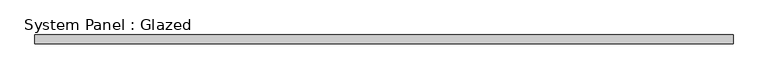
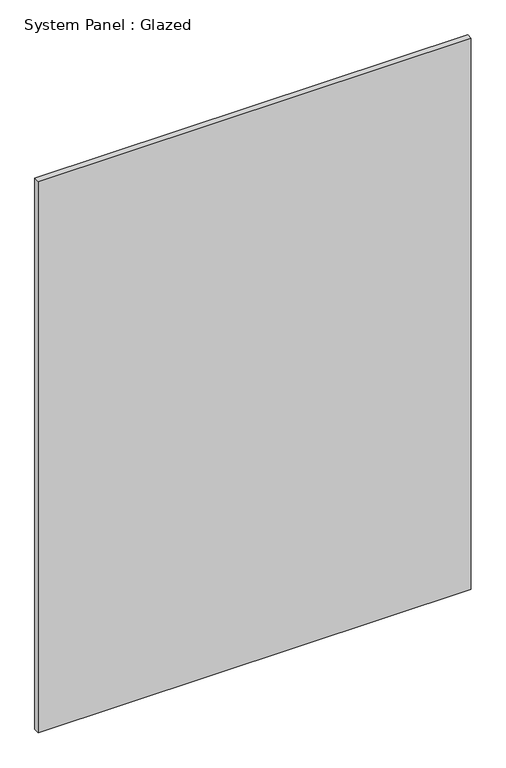
"""IFC4 building model written with IfcOpenShell, lengths in millimetres: plate geometry, System Panel : Glazed."""

from ifc_helpers import new_model, si_unit, origin, origin_with_axes, place, context, project, spatial, polyline, outline, extrude, source, transform, mapped, element, save


def system_panel_glazed_321bf09d(model_context):
    return source(origin(), model_context, "Body", "SweptSolid", [
        extrude(outline(polyline([(975.0, 24.5), (-975.0, 24.5), (-975.0, 49.5), (975.0, 49.5), (975.0, 24.5)])), origin_with_axes(), (0.0, 0.0, 1.0), 2625.0),
    ])


if __name__ == "__main__":
    model = new_model("IFC4")
    model_context = context("Model", 3, world=origin())
    ifc_project = project(units=[si_unit("LENGTHUNIT", "METRE", prefix="MILLI")], contexts=[model_context])
    site = spatial("IfcSite", under=ifc_project)
    building = spatial("IfcBuilding", under=site)
    placement = place(None, origin())
    system_panel_glazed_shape = system_panel_glazed_321bf09d(model_context)
    element("IfcPlate", 1, ObjectType="System Panel : Glazed", at=placement, inside=building, context=model_context, shape_type="MappedRepresentation", body=[
        mapped(system_panel_glazed_shape, transform((0.0, 0.0, 0.0), x_axis=(1.0, 0.0, 0.0), y_axis=(0.0, 1.0, 0.0), z_axis=(0.0, 0.0, 1.0))),
    ])
    save(model, "model.ifc")

# Revit data of these elements
# Element 1 (IfcPlate, "System Panel : Glazed")
#   Materials on its faces: "Glass"
# Materials
#   "Glass": class "Glass", colour RGB 0 128 192, transparency 0.9
